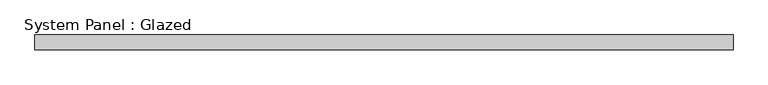
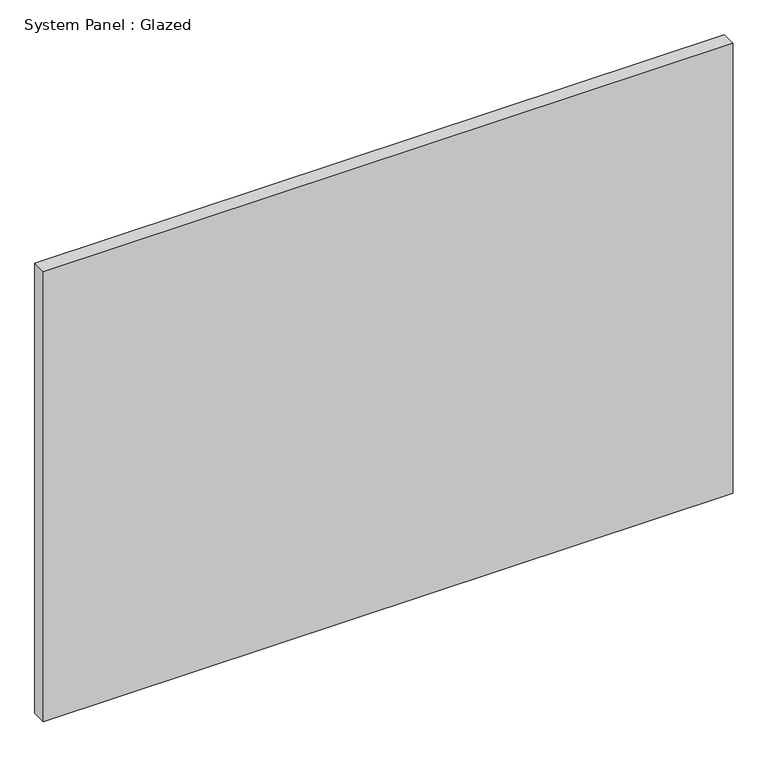
"""IFC4 building model written with IfcOpenShell, lengths in millimetres: plate geometry, System Panel : Glazed."""

import ifcopenshell
import ifcopenshell.guid

model = None  # the IFC model being written
_history = None  # IfcOwnerHistory: only IFC2X3 demands one
_inside = {}  # id of a spatial element -> (the spatial element, [elements in it])
_under = {}  # id of a project, library or spatial element -> (it, [spatial elements below it])
_declared = {}  # id of a project -> (the project, [libraries it declares])
_typed = {}  # id of a type object -> (the type object, [elements of that type])
_made_of = {}  # id of a material, layer set ... -> (it, [elements and type objects made of it])


def new_model(schema):
    """Start an empty IFC model of exactly this schema.

    Asked for "IFC4X3", IfcOpenShell would pick the latest addendum, in which some entities
    have other attributes; the version numbers below select the first issue.
    IFC2X3 requires an IfcOwnerHistory on every rooted entity: one is made here for all.
    """
    global model, _history
    if schema == "IFC4X3":
        model = ifcopenshell.file(schema_version=(4, 3, 0, 0))
    else:
        model = ifcopenshell.file(schema=schema)
    _inside.clear()
    _under.clear()
    _declared.clear()
    _typed.clear()
    _made_of.clear()
    _history = None
    if model.schema == "IFC2X3":
        org = make("IfcOrganization", Name="unknown")
        user = make(
            "IfcPersonAndOrganization",
            ThePerson=make("IfcPerson", FamilyName="unknown"),
            TheOrganization=org,
        )
        app = make(
            "IfcApplication",
            ApplicationDeveloper=org,
            Version="unknown",
            ApplicationFullName="unknown",
            ApplicationIdentifier="unknown",
        )
        _history = make(
            "IfcOwnerHistory",
            OwningUser=user,
            OwningApplication=app,
            ChangeAction="ADDED",
            CreationDate=0,
        )
    return model


def make(cls, **values):
    """One entity of the class cls with the attributes given. An attribute that is None is left unset."""
    return model.create_entity(
        cls, **{name: value for name, value in values.items() if value is not None}
    )


def rooted(cls, **values):
    """An entity with a GlobalId (a new one), such as an element, a storey or a relation."""
    return make(cls, GlobalId=ifcopenshell.guid.new(), OwnerHistory=_history, **values)


def si_unit(unit_type, name, prefix=None):
    """IfcSIUnit, for example si_unit("LENGTHUNIT", "METRE", prefix="MILLI")."""
    return make("IfcSIUnit", UnitType=unit_type, Prefix=prefix, Name=name)


def assignment(units):
    """IfcUnitAssignment: the units of a project."""
    return None if units is None else make("IfcUnitAssignment", Units=units)


def point(xyz):
    """IfcCartesianPoint."""
    return None if xyz is None else make("IfcCartesianPoint", Coordinates=xyz)


def direction(xyz):
    """IfcDirection."""
    return None if xyz is None else make("IfcDirection", DirectionRatios=xyz)


def frame(location, z_axis=None, x_axis=None):
    """IfcAxis2Placement3D, a coordinate frame: its origin and axes. An axis left out is left unset."""
    return make(
        "IfcAxis2Placement3D",
        Location=point(location),
        Axis=direction(z_axis),
        RefDirection=direction(x_axis),
    )


def origin():
    """The frame at (0, 0, 0) with its axes left unset."""
    return frame((0.0, 0.0, 0.0))


def origin_with_axes():
    """The frame at (0, 0, 0) with the z axis (0, 0, 1) and the x axis (1, 0, 0) written out."""
    return frame((0.0, 0.0, 0.0), z_axis=(0.0, 0.0, 1.0), x_axis=(1.0, 0.0, 0.0))


def place(relative_to, where):
    """IfcLocalPlacement: puts the frame where relative to a parent placement (None: the world)."""
    return make(
        "IfcLocalPlacement", PlacementRelTo=relative_to, RelativePlacement=where
    )


def context(
    kind, dimensions, precision=None, world=None, true_north=None, identifier=None
):
    """IfcGeometricRepresentationContext, for example the 3D "Model" context."""
    return make(
        "IfcGeometricRepresentationContext",
        ContextIdentifier=identifier,
        ContextType=kind,
        CoordinateSpaceDimension=dimensions,
        Precision=precision,
        WorldCoordinateSystem=world,
        TrueNorth=true_north,
    )


def project(units=None, contexts=None):
    """IfcProject with its units and contexts."""
    return rooted(
        "IfcProject",
        Name="project",
        RepresentationContexts=contexts,
        UnitsInContext=assignment(units),
    )


def spatial(cls, under=None, at=None, **own):
    """A site, building, storey or space (cls), placed at a placement, below another one or the project."""
    s = rooted(cls, ObjectPlacement=at, **own)
    if under is not None:
        _under.setdefault(under.id(), (under, []))[1].append(s)
    return s


def polyline(points):
    """IfcPolyline through the points."""
    return make("IfcPolyline", Points=[point(p) for p in points])


def outline(outer, holes=None, kind="AREA"):
    """IfcArbitraryClosedProfileDef: a profile drawn as a closed curve; with holes, ...WithVoids."""
    if holes is None:
        return make("IfcArbitraryClosedProfileDef", ProfileType=kind, OuterCurve=outer)
    return make(
        "IfcArbitraryProfileDefWithVoids",
        ProfileType=kind,
        OuterCurve=outer,
        InnerCurves=holes,
    )


def extrude(swept, where, along, depth):
    """IfcExtrudedAreaSolid: the profile swept, set in the frame where, extruded along a direction by depth."""
    return make(
        "IfcExtrudedAreaSolid",
        SweptArea=swept,
        Position=where,
        ExtrudedDirection=direction(along),
        Depth=depth,
    )


def shape(context_of_items, identifier, shape_type, items):
    """IfcShapeRepresentation: the items that make up one representation, for example the "Body"."""
    return make(
        "IfcShapeRepresentation",
        ContextOfItems=context_of_items,
        RepresentationIdentifier=identifier,
        RepresentationType=shape_type,
        Items=items,
    )


def source(mapping_origin, context_of_items, identifier, shape_type, items):
    """IfcRepresentationMap: a shape defined once, which mapped items show again and again."""
    return make(
        "IfcRepresentationMap",
        MappingOrigin=mapping_origin,
        MappedRepresentation=shape(context_of_items, identifier, shape_type, items),
    )


def transform(
    local_origin,
    x_axis=None,
    y_axis=None,
    z_axis=None,
    scale=None,
    scale2=None,
    scale3=None,
    uniform=True,
):
    """IfcCartesianTransformationOperator3D, or its non-uniform kind. x_axis, y_axis, z_axis: its Axis1, 2, 3."""
    if uniform:
        return make(
            "IfcCartesianTransformationOperator3D",
            Axis1=direction(x_axis),
            Axis2=direction(y_axis),
            LocalOrigin=point(local_origin),
            Scale=scale,
            Axis3=direction(z_axis),
        )
    return make(
        "IfcCartesianTransformationOperator3DnonUniform",
        Axis1=direction(x_axis),
        Axis2=direction(y_axis),
        LocalOrigin=point(local_origin),
        Scale=scale,
        Axis3=direction(z_axis),
        Scale2=scale2,
        Scale3=scale3,
    )


def mapped(mapping_source, mapping_target):
    """IfcMappedItem: shows the shape of a source again, moved by a transform."""
    return make(
        "IfcMappedItem", MappingSource=mapping_source, MappingTarget=mapping_target
    )


def made_of(thing, what):
    """Note that an element or type object is made of a material, layer set ...; save() writes the relation."""
    if what is not None:
        _made_of.setdefault(what.id(), (what, []))[1].append(thing)
    return thing


def element(
    cls,
    number,
    at=None,
    inside=None,
    cuts=None,
    type_object=None,
    material=None,
    context=None,
    identifier="Body",
    shape_type=None,
    held_by="IfcProductDefinitionShape",
    body=None,
    shapes=None,
    **own,
):
    """One element of the class cls, such as IfcWall. Its Tag is "e" and its number.

    at: its placement. inside: the storey or other place that contains it. cuts: it is an
    opening in that element (IfcRelVoidsElement). A single representation is given by context,
    identifier, shape_type and body (its items); several are given by shapes. held_by: the class
    of the entity that holds the representations. save() writes the other relations.
    """
    e = rooted(cls, Tag="e%d" % number, ObjectPlacement=at, **own)
    if body is not None:
        shapes = [shape(context, identifier, shape_type, body)]
    if shapes is not None:
        e.Representation = make(held_by, Representations=shapes)
    if inside is not None:
        _inside.setdefault(inside.id(), (inside, []))[1].append(e)
    if cuts is not None:
        rooted(
            "IfcRelVoidsElement", RelatingBuildingElement=cuts, RelatedOpeningElement=e
        )
    if type_object is not None:
        _typed.setdefault(type_object.id(), (type_object, []))[1].append(e)
    return made_of(e, material)


def aggregate(whole, parts):
    """IfcRelAggregates: a whole, such as a stair, and the parts it consists of."""
    return rooted("IfcRelAggregates", RelatingObject=whole, RelatedObjects=parts)


def save(model, path):
    """Write the relations noted so far, then the file.

    IfcRelAggregates (storeys below a building ...), IfcRelContainedInSpatialStructure (elements
    in a storey), IfcRelDefinesByType, IfcRelAssociatesMaterial and IfcRelDeclares: one each for
    every whole, place, type object, material and project.
    """
    for whole, parts in _under.values():
        aggregate(whole, parts)
    for where, things in _inside.values():
        rooted(
            "IfcRelContainedInSpatialStructure",
            RelatedElements=things,
            RelatingStructure=where,
        )
    for kind, things in _typed.values():
        rooted("IfcRelDefinesByType", RelatedObjects=things, RelatingType=kind)
    for what, things in _made_of.values():
        rooted("IfcRelAssociatesMaterial", RelatedObjects=things, RelatingMaterial=what)
    for by, libraries in _declared.values():
        rooted("IfcRelDeclares", RelatingContext=by, RelatedDefinitions=libraries)
    model.write(path)


def system_panel_glazed_2ccc015e(model_context):
    return source(origin(), model_context, "Body", "SweptSolid", [
        extrude(outline(polyline([(593.725, 19.05), (-593.725, 19.05), (-593.725, 44.45), (593.725, 44.45), (593.725, 19.05)])), origin_with_axes(), (0.0, 0.0, 1.0), 819.15),
    ])


if __name__ == "__main__":
    model = new_model("IFC4")
    model_context = context("Model", 3, world=origin())
    ifc_project = project(units=[si_unit("LENGTHUNIT", "METRE", prefix="MILLI")], contexts=[model_context])
    site = spatial("IfcSite", under=ifc_project)
    building = spatial("IfcBuilding", under=site)
    placement = place(None, origin())
    system_panel_glazed_shape = system_panel_glazed_2ccc015e(model_context)
    element("IfcPlate", 1, ObjectType="System Panel : Glazed", at=placement, inside=building, context=model_context, shape_type="MappedRepresentation", body=[
        mapped(system_panel_glazed_shape, transform((0.0, 0.0, 0.0), x_axis=(1.0, 0.0, 0.0), y_axis=(0.0, 1.0, 0.0), z_axis=(0.0, 0.0, 1.0))),
    ])
    save(model, "model.ifc")

# Revit data of these elements
# Type "System Panel : Glazed"
#   Construction Type Id = "GSP4R"
#   Analytic Construction = "1/8 in Pilkington single glazing"
#   Visual Light Transmittance = 0.9
#   Solar Heat Gain Coefficient = 0.86
#   Heat Transfer Coefficient (U) = 1.18115 BTU/(h·ft²·°F)
#   Define Thermal Properties by = 1
# Element 1 (IfcPlate, "System Panel : Glazed")
#   Materials on its faces: "Glass"
# Materials
#   "Glass": class "Glass", colour RGB 0 128 192, transparency 0.75, Description = "Soda Lime Glass", Cost = 0
